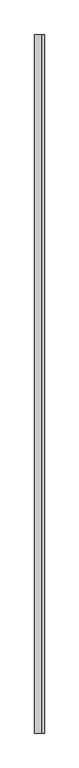
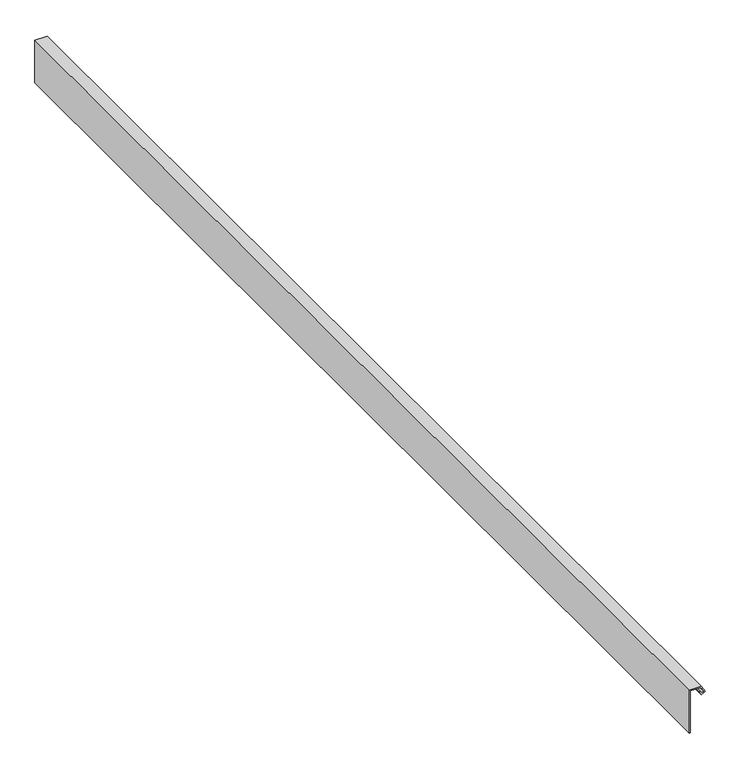
"""IFC4 building model written with IfcOpenShell, lengths in millimetres: proxy geometry, Flashing10:Flashing020:293153 : Flashing10:Flashing020:293153."""

from ifc_helpers import new_model, si_unit, frame, origin, place, context, project, spatial, polyline, outline, extrude, source, transform, mapped, element, save


def generic_models_23ae902f(model_context):
    return source(origin(), model_context, "Body", "SweptSolid", [
        extrude(outline(polyline([(40707.8367187, 21407.337233), (40707.8367187, 21409.337233), (40785.71875, 21409.337233), (40785.71875, 21427.5312589), (40777.2623654, 21432.3078529), (40775.2340727, 21429.1698105), (40779.327926, 21426.9629677), (40778.3789062, 21425.2024674), (40772.3789062, 21428.4368424), (40776.6054687, 21434.9759049), (40787.71875, 21428.6985611), (40787.71875, 21407.337233), (40707.8367187, 21407.337233)])), frame((0.0, 8260.4774523, 0.0), z_axis=(0.0, 1.0, 0.0), x_axis=(0.0, 0.0, 1.0)), (0.0, 0.0, 1.0), 2000.0),
    ])


if __name__ == "__main__":
    model = new_model("IFC4")
    model_context = context("Model", 3, world=origin())
    ifc_project = project(units=[si_unit("LENGTHUNIT", "METRE", prefix="MILLI")], contexts=[model_context])
    site = spatial("IfcSite", under=ifc_project)
    building = spatial("IfcBuilding", under=site)
    placement = place(None, origin())
    generic_models_shape = generic_models_23ae902f(model_context)
    element("IfcBuildingElementProxy", 1, Name="Flashing10:Flashing020:293153 : Flashing10:Flashing020:293153", ObjectType="Flashing10:Flashing020:293153 : Flashing10:Flashing020:293153", at=placement, inside=building, context=model_context, shape_type="MappedRepresentation", body=[
        mapped(generic_models_shape, transform((0.0, 0.0, 0.0), x_axis=(1.0, 0.0, 0.0), y_axis=(0.0, 1.0, 0.0), z_axis=(0.0, 0.0, 1.0))),
    ])
    save(model, "model.ifc")

# Revit data of these elements
# Type "Flashing10:Flashing020:293153 : Flashing10:Flashing020:293153"
#   NameOverride = "Flashing10:Flashing020:293153"
#   ObjectTypeOverride = "Flashing10:Flashing020"
#   Reference = "Flashing020"
#   Category = "Generic Models"
#   Tag = "293153"
# Element 1 (IfcBuildingElementProxy, "Flashing10:Flashing020:293153 : Flashing10:Flashing020:293153")
#   Materials on its faces: "BRAKE METAL TO WRAP FRAMING OVER BITUTHANE"
# Materials
#   "BRAKE METAL TO WRAP FRAMING OVER BITUTHANE": class "Unassigned", colour RGB 128 128 128, transparency 0, Cost = 0
